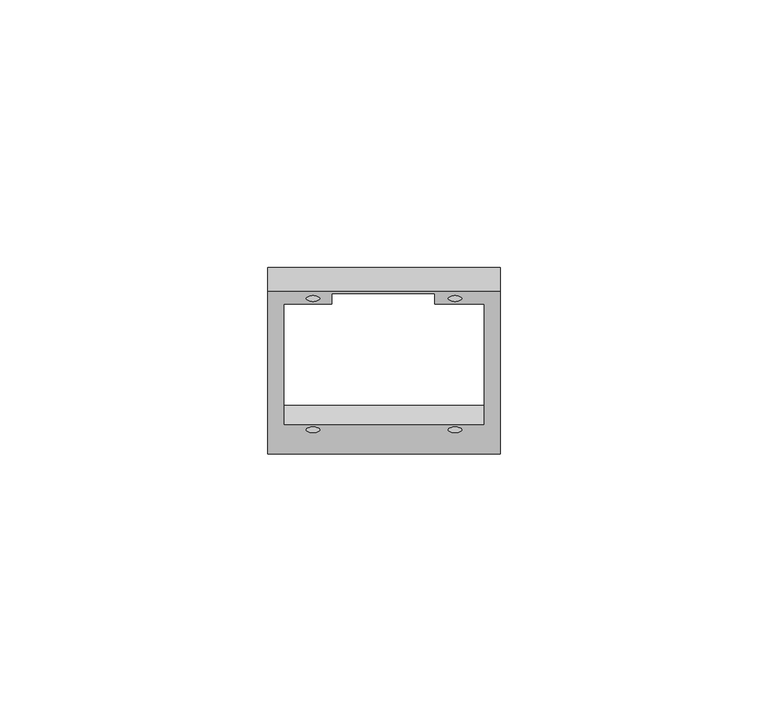
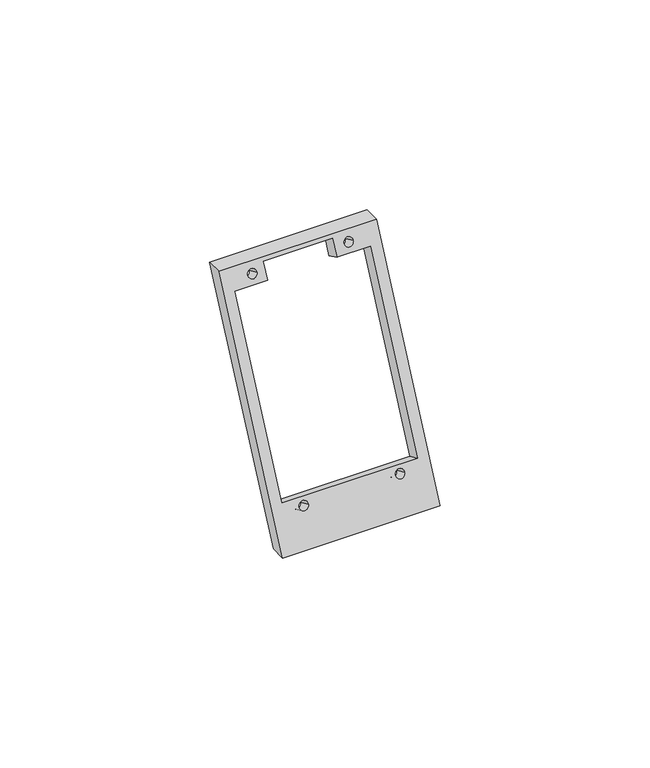
"""IFC4 building model written with IfcOpenShell, lengths in millimetres: furniture geometry, MOLDURA TELA : MOLDURA TELA."""

from ifc_helpers import new_model, si_unit, frame, origin, place, context, project, spatial, polyline, circle_curve, source, transform, mapped, element, save
from ifc_brep_helpers import plane_surface, revolved_surface, advanced_brep


def furniture_6c0b4a62(model_context):
    return source(origin(), model_context, "Body", "AdvancedBrep", [
        advanced_brep(
        [(2369.0719295, 1292.0509228, 0.0), (2369.0719295, 1322.3609206, 65.0), (2412.3719295, 1322.3609206, 65.0), (2412.3719295, 1292.0509228, 0.0), (2402.7219295, 1320.2478293, 60.4684611), (2405.2219295, 1320.2478293, 60.4684611), (2409.3719295, 1296.7079921, 9.9871173), (2409.3719295, 1319.10676, 58.02143), (2400.0719295, 1319.10676, 58.02143), (2400.0719295, 1321.0930658, 62.2810766), (2381.0719295, 1321.0930658, 62.2810766), (2381.0719295, 1319.10676, 58.02143), (2372.0719295, 1319.10676, 58.02143), (2372.0719295, 1296.7079921, 9.9871173), (2405.2219295, 1295.7359701, 7.9026094), (2402.7219295, 1295.7359701, 7.9026094), (2378.7219295, 1295.7359701, 7.9026094), (2376.2219295, 1295.7359701, 7.9026094), (2378.7219295, 1320.2478293, 60.4684611), (2376.2219295, 1320.2478293, 60.4684611), (2412.3719295, 1287.6374112, 0.0), (2412.3719295, 1317.9474089, 65.0), (2369.0719295, 1317.9474089, 65.0), (2369.0719295, 1287.6374112, 0.0), (2402.7219295, 1316.6225981, 62.1589341), (2405.2219295, 1316.6225981, 62.1589341), (2409.3719295, 1293.082761, 11.6775904), (2372.0719295, 1293.082761, 11.6775904), (2372.0719295, 1315.4815288, 59.7119031), (2381.0719295, 1315.4815288, 59.7119031), (2381.0719295, 1317.4678347, 63.9715497), (2400.0719295, 1317.4678347, 63.9715497), (2400.0719295, 1315.4815288, 59.7119031), (2409.3719295, 1315.4815288, 59.7119031), (2405.2219295, 1292.110739, 9.5930825), (2402.7219295, 1292.110739, 9.5930825), (2378.7219295, 1292.110739, 9.5930825), (2376.2219295, 1292.110739, 9.5930825), (2378.7219295, 1316.6225981, 62.1589341), (2376.2219295, 1316.6225981, 62.1589341)],
        [
            (0, 1),
            (1, 2),
            (2, 3),
            (3, 0),
            (4, 5, circle_curve(frame((2403.9719295, 1320.2478293, 60.4684611), z_axis=(0.0, -0.9063077870366535, 0.4226182617406919), x_axis=(-1.0, 0.0, 0.0)), 1.25)),
            (5, 4, circle_curve(frame((2403.9719295, 1320.2478293, 60.4684611), z_axis=(0.0, -0.9063077870366535, 0.4226182617406919), x_axis=(-1.0, 0.0, 0.0)), 1.25)),
            (6, 7),
            (7, 8),
            (8, 9),
            (9, 10),
            (10, 11),
            (11, 12),
            (12, 13),
            (13, 6),
            (14, 15, circle_curve(frame((2403.9719295, 1295.7359701, 7.9026094), z_axis=(0.0, -0.9063077870366535, 0.4226182617406919), x_axis=(-1.0, 0.0, 0.0)), 1.25)),
            (15, 14, circle_curve(frame((2403.9719295, 1295.7359701, 7.9026094), z_axis=(0.0, -0.9063077870366535, 0.4226182617406919), x_axis=(-1.0, 0.0, 0.0)), 1.25)),
            (16, 17, circle_curve(frame((2377.4719295, 1295.7359701, 7.9026094), z_axis=(0.0, -0.9063077870366535, 0.4226182617406919), x_axis=(1.0, 0.0, 0.0)), 1.25)),
            (17, 16, circle_curve(frame((2377.4719295, 1295.7359701, 7.9026094), z_axis=(0.0, -0.9063077870366535, 0.4226182617406919), x_axis=(1.0, 0.0, 0.0)), 1.25)),
            (18, 19, circle_curve(frame((2377.4719295, 1320.2478293, 60.4684611), z_axis=(0.0, -0.9063077870366535, 0.4226182617406919), x_axis=(1.0, 0.0, 0.0)), 1.25)),
            (19, 18, circle_curve(frame((2377.4719295, 1320.2478293, 60.4684611), z_axis=(0.0, -0.9063077870366535, 0.4226182617406919), x_axis=(1.0, 0.0, 0.0)), 1.25)),
            (20, 21),
            (21, 22),
            (22, 23),
            (23, 20),
            (24, 25, circle_curve(frame((2403.9719295, 1316.6225981, 62.1589341), z_axis=(0.0, 0.9063077870366535, -0.4226182617406919), x_axis=(-1.0, 0.0, 0.0)), 1.25)),
            (25, 24, circle_curve(frame((2403.9719295, 1316.6225981, 62.1589341), z_axis=(0.0, 0.9063077870366535, -0.4226182617406919), x_axis=(-1.0, 0.0, 0.0)), 1.25)),
            (26, 27),
            (27, 28),
            (28, 29),
            (29, 30),
            (30, 31),
            (31, 32),
            (32, 33),
            (33, 26),
            (34, 35, circle_curve(frame((2403.9719295, 1292.110739, 9.5930825), z_axis=(0.0, 0.9063077870366535, -0.4226182617406919), x_axis=(-1.0, 0.0, 0.0)), 1.25)),
            (35, 34, circle_curve(frame((2403.9719295, 1292.110739, 9.5930825), z_axis=(0.0, 0.9063077870366535, -0.4226182617406919), x_axis=(-1.0, 0.0, 0.0)), 1.25)),
            (36, 37, circle_curve(frame((2377.4719295, 1292.110739, 9.5930825), z_axis=(0.0, 0.9063077870366535, -0.4226182617406919), x_axis=(1.0, 0.0, 0.0)), 1.25)),
            (37, 36, circle_curve(frame((2377.4719295, 1292.110739, 9.5930825), z_axis=(0.0, 0.9063077870366535, -0.4226182617406919), x_axis=(1.0, 0.0, 0.0)), 1.25)),
            (38, 39, circle_curve(frame((2377.4719295, 1316.6225981, 62.1589341), z_axis=(0.0, 0.9063077870366535, -0.4226182617406919), x_axis=(1.0, 0.0, 0.0)), 1.25)),
            (39, 38, circle_curve(frame((2377.4719295, 1316.6225981, 62.1589341), z_axis=(0.0, 0.9063077870366535, -0.4226182617406919), x_axis=(1.0, 0.0, 0.0)), 1.25)),
            (0, 23),
            (22, 1),
            (2, 21),
            (20, 3),
            (4, 24),
            (25, 5),
            (6, 26),
            (33, 7),
            (32, 8),
            (31, 9),
            (30, 10),
            (29, 11),
            (28, 12),
            (27, 13),
            (14, 34),
            (35, 15),
            (16, 36),
            (37, 17),
            (18, 38),
            (39, 19),
        ],
        [
            plane_surface(frame((2369.0719295, 1293.6228788, 3.3710705), z_axis=(0.0, 0.9063077870366535, -0.4226182617406919), x_axis=(0.0, 0.4226182617406919, 0.9063077870366535))),
            plane_surface(frame((2369.0719295, 1289.9976477, 5.0615435), z_axis=(0.0, -0.9063077870366535, 0.4226182617406919), x_axis=(0.0, -0.4226182617406919, -0.9063077870366535))),
            plane_surface(frame((2369.0719295, 1290.6199639, -3.0687014), z_axis=(-1.0, 0.0, 0.0), x_axis=(0.0, -0.9063077870366527, 0.42261826174069356))),
            plane_surface(frame((2412.3719295, 1322.3609206, 65.0), z_axis=(1.0, 0.0, 0.0), x_axis=(0.0, -0.9063077870366535, 0.42261826174069184))),
            revolved_surface(polyline([(2402.7219295, 1316.6225981272491, 62.15893415843589), (2402.7219295, 1320.2478293, 60.4684611)]), (2403.9719295, 1320.2478293, 60.4684611), (0.0, -0.9063077870366535, 0.4226182617406919)),
            plane_surface(frame((2409.3719295, 1296.7079921, 9.9871173), z_axis=(-1.0, 0.0, 0.0), x_axis=(0.0, -0.9063077870366532, 0.4226182617406927))),
            plane_surface(frame((2409.3719295, 1319.10676, 58.02143), z_axis=(0.0, -0.42261826174069184, -0.9063077870366535), x_axis=(0.0, -0.9063077870366535, 0.42261826174069184))),
            plane_surface(frame((2400.0719295, 1319.10676, 58.02143), z_axis=(-1.0, 0.0, 0.0), x_axis=(0.0, -0.9063077870366535, 0.42261826174069184))),
            plane_surface(frame((2400.0719295, 1321.0930658, 62.2810766), z_axis=(0.0, -0.42261826174069184, -0.9063077870366535), x_axis=(0.0, -0.9063077870366535, 0.42261826174069184))),
            plane_surface(frame((2381.0719295, 1321.0930658, 62.2810766), z_axis=(1.0, 0.0, 0.0), x_axis=(0.0, -0.9063077870366527, 0.42261826174069356))),
            plane_surface(frame((2381.0719295, 1319.10676, 58.02143), z_axis=(0.0, -0.42261826174069184, -0.9063077870366535), x_axis=(0.0, -0.9063077870366535, 0.42261826174069184))),
            plane_surface(frame((2372.0719295, 1319.10676, 58.02143), z_axis=(1.0, 0.0, 0.0), x_axis=(0.0, -0.9063077870366535, 0.42261826174069184))),
            plane_surface(frame((2372.0719295, 1296.7079921, 9.9871173), z_axis=(0.0, 0.4226182617406927, 0.9063077870366532), x_axis=(0.0, -0.9063077870366532, 0.4226182617406927))),
            revolved_surface(polyline([(2402.7219295, 1292.1107389710862, 9.593082437994347), (2402.7219295, 1295.7359701, 7.9026094)]), (2403.9719295, 1295.7359701, 7.9026094), (0.0, -0.9063077870366535, 0.4226182617406919)),
            revolved_surface(polyline([(2378.7219295, 1292.1107389710862, 9.593082437994347), (2378.7219295, 1295.7359701, 7.9026094)]), (2377.4719295, 1295.7359701, 7.9026094), (0.0, -0.9063077870366535, 0.4226182617406919)),
            revolved_surface(polyline([(2378.7219295, 1316.6225981272491, 62.15893415843589), (2378.7219295, 1320.2478293, 60.4684611)]), (2377.4719295, 1320.2478293, 60.4684611), (0.0, -0.9063077870366535, 0.4226182617406919)),
            plane_surface(frame((2418.7000554, 1312.6608189, 65.0), z_axis=(0.0, 0.0, 1.0), x_axis=(-1.0, 0.0, 0.0))),
            plane_surface(frame((2418.7000554, 1302.9468274, 0.0), z_axis=(0.0, 0.0, -1.0), x_axis=(-1.0, 0.0, 0.0))),
        ],
        [
            (0, [[1, 2, 3, 4], [5, 6], [7, 8, 9, 10, 11, 12, 13, 14], [15, 16], [17, 18], [19, 20]]),
            (1, [[21, 22, 23, 24], [25, 26], [27, 28, 29, 30, 31, 32, 33, 34], [35, 36], [37, 38], [39, 40]]),
            (2, [[-1, 41, -23, 42]]),
            (3, [[-3, 43, -21, 44]]),
            (4, [[-5, 45, -26, 46]]),
            (4, [[-6, -46, -25, -45]]),
            (5, [[-7, 47, -34, 48]]),
            (6, [[-8, -48, -33, 49]]),
            (7, [[-9, -49, -32, 50]]),
            (8, [[-10, -50, -31, 51]]),
            (9, [[-11, -51, -30, 52]]),
            (10, [[-12, -52, -29, 53]]),
            (11, [[-13, -53, -28, 54]]),
            (12, [[-14, -54, -27, -47]]),
            (13, [[-15, 55, -36, 56]]),
            (13, [[-16, -56, -35, -55]]),
            (14, [[-17, 57, -38, 58]]),
            (14, [[-18, -58, -37, -57]]),
            (15, [[-19, 59, -40, 60]]),
            (15, [[-20, -60, -39, -59]]),
            (16, [[-2, -42, -22, -43]]),
            (17, [[-4, -44, -24, -41]]),
        ],
    ),
    ])


if __name__ == "__main__":
    model = new_model("IFC4")
    model_context = context("Model", 3, world=origin())
    ifc_project = project(units=[si_unit("LENGTHUNIT", "METRE", prefix="MILLI")], contexts=[model_context])
    site = spatial("IfcSite", under=ifc_project)
    building = spatial("IfcBuilding", under=site)
    placement = place(None, origin())
    furniture_shape = furniture_6c0b4a62(model_context)
    element("IfcFurniture", 1, ObjectType="MOLDURA TELA : MOLDURA TELA", at=placement, inside=building, context=model_context, shape_type="MappedRepresentation", body=[
        mapped(furniture_shape, transform((0.0, 0.0, 0.0), x_axis=(1.0, 0.0, 0.0), y_axis=(0.0, 1.0, 0.0), z_axis=(0.0, 0.0, 1.0))),
    ])
    save(model, "model.ifc")

# Revit data of these elements
# Type "MOLDURA TELA : MOLDURA TELA"
#   Height = 0
# Element 1 (IfcFurniture, "MOLDURA TELA : MOLDURA TELA")
#   Materials on its faces: ".BOX FUNDO"
# Materials
#   ".BOX FUNDO": class "Vidro", colour RGB 236 240 239, transparency 0.15, Cost = 0
